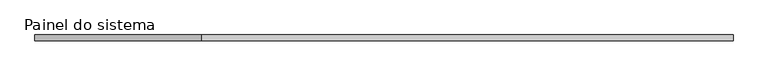
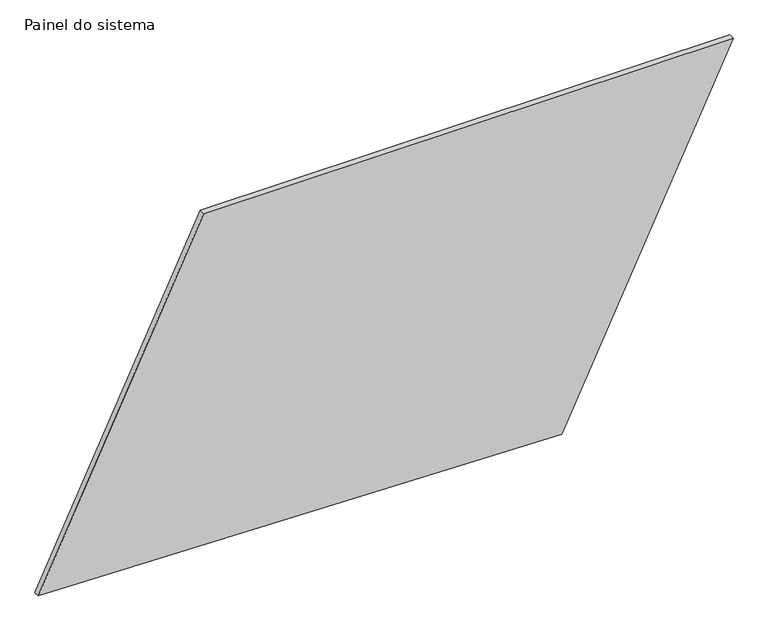
"""IFC4 building model written with IfcOpenShell, lengths in millimetres: plate geometry, Painel do sistema : Envidraçado."""

from ifc_helpers import new_model, si_unit, frame, origin, place, context, project, spatial, polyline, outline, extrude, source, transform, mapped, element, save


def painel_do_sistema_79c66f50(model_context):
    return source(origin(), model_context, "Body", "SweptSolid", [
        extrude(outline(polyline([(53.7655622, -1498.9957573), (0.0, 760.0687219), (1547.9439006, 1498.9957573), (1547.9439006, -785.7342692), (53.7655622, -1498.9957573)])), frame((0.0, 24.5, 0.0), z_axis=(0.0, 1.0, 0.0), x_axis=(0.0, 0.0, 1.0)), (0.0, 0.0, 1.0), 25.0),
    ])


if __name__ == "__main__":
    model = new_model("IFC4")
    model_context = context("Model", 3, world=origin())
    ifc_project = project(units=[si_unit("LENGTHUNIT", "METRE", prefix="MILLI")], contexts=[model_context])
    site = spatial("IfcSite", under=ifc_project)
    building = spatial("IfcBuilding", under=site)
    placement = place(None, origin())
    painel_do_sistema_shape = painel_do_sistema_79c66f50(model_context)
    element("IfcPlate", 1, ObjectType="Painel do sistema : Envidraçado", at=placement, inside=building, context=model_context, shape_type="MappedRepresentation", body=[
        mapped(painel_do_sistema_shape, transform((0.0, 0.0, 0.0), x_axis=(1.0, 0.0, 0.0), y_axis=(0.0, 1.0, 0.0), z_axis=(0.0, 0.0, 1.0))),
    ])
    save(model, "model.ifc")

# Revit data of these elements
# Type "Painel do sistema : Envidraçado"
#   Construction Type Id = "GSP4R"
#   Analytic Construction = "Vidraça única Pilkington 1/8 pol"
#   Visual Light Transmittance = 0.9
#   Solar Heat Gain Coefficient = 0.86
#   Heat Transfer Coefficient (U) = 6.7069 W/(m²·K)
# Element 1 (IfcPlate, "Painel do sistema : Envidraçado")
#   Materials on its faces: "Vidro"
# Materials
#   "Vidro": class "Vidro", colour RGB 0 128 192, transparency 0.9, Description = "Vidro de sílica", Cost = 0
